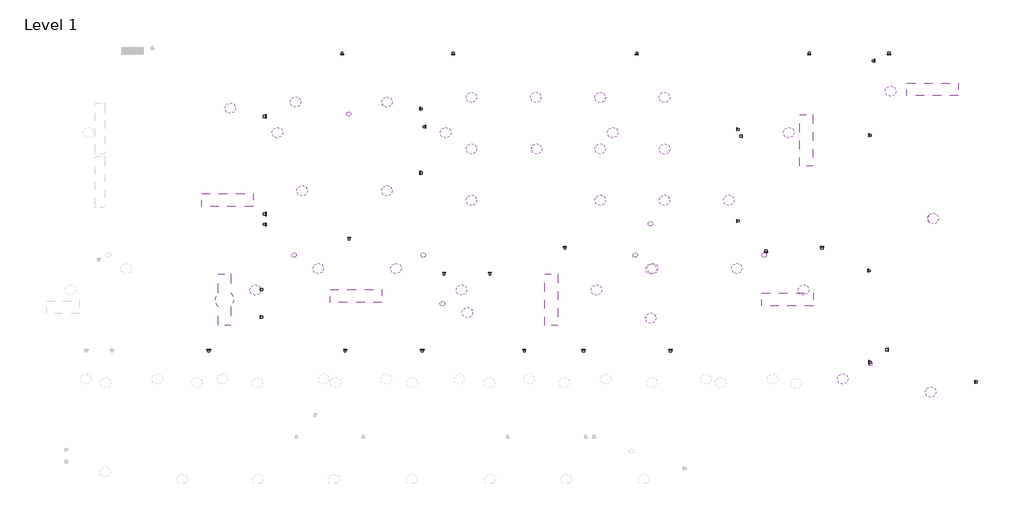
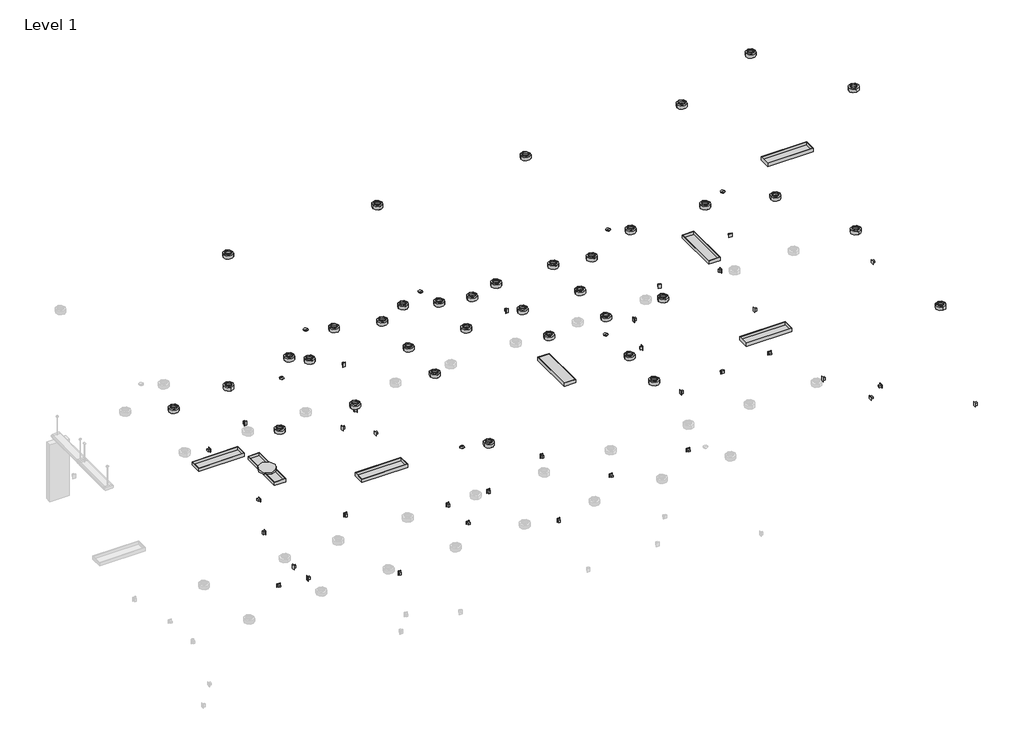
# One storey, part 3 of 3: 43 light fixtures, 22 proxies, 20 switching devices.
# Revit data of these elements (continued)
# Project information
#   Author = "F.W."
#   Classification.Facility.Description = "Mixed-Gender Dormitory"
#   Classification.Facility.Number = "11-16 27 14"
#   COBie.CreatedBy = "info@mma.ie"
#   COBie.CreatedOn = "2017-07-25T10:15:16"
#   COBie.Facility.Name = "EDTP-001"
#   COBie.Facility.Category = "11-16 27 14 : Mixed-Gender Dormitory"
#   COBie.Facility.ProjectName = "East Dormitory Project"
#   COBie.Facility.SiteName = "East Healey Street, Champaign, Illiniois USA"
#   COBie.Facility.LinearUnits = "Millimeters"
#   COBie.Facility.AreaUnits = "Square Meters"
#   COBie.Facility.VolumeUnits = "Cubic Meters"
#   COBie.Facility.CurrencyUnit = "Dollar"
#   COBie.Facility.AreaMeasurement = "Revit Default Area Calculation Method"
#   COBie.Facility.Description = "Two Story, Luxury Dormitory"
#   COBie.Facility.ProjectDescription = "One of Four Dormitories on the E.Healey Site"
#   COBie.Facility.SiteDescription = "Four Dormitories Project Site"
#   COBie.Facility.Phase = "60% Design Submission"
#   Project Issue Date = "Issue Date"
#   Project Status = "Final Issue"
#   Client Name = "Prairie Sky Consulting"
#   Project Address = "East Healey Street,\nChampaign,\nIllinois,\nUSA."
#   Project Name = "Four Dormitory Complex"
#   Project Number = "East Dormitory"
# Grids (mm)
#   "1": line (0.005, 17313.813) -> (0.005, -2035.285)
#   "A": line (-2283.993, 15250.039) -> (37015.009, 15250.039)
#   "B": line (37015.009, 12550.039) -> (-2283.993, 12550.039)
#   "C": line (37015.009, 6550.039) -> (-2283.993, 6550.039)
#   "D": line (37015.009, 2000.039) -> (-2523.993, 2000.039)
#   "E": line (37015.009, 0.039) -> (-2283.993, 0.039)
#   "2": line (1900.005, 17313.813) -> (1900.005, -2035.285)
#   "3": line (5650.005, 17313.813) -> (5650.005, -2035.285)
#   "4": line (8350.005, 17313.813) -> (8350.005, -2035.285)
#   "6": line (28050.005, -2035.285) -> (28050.005, 17313.813)
#   "8": line (34850.005, -2035.285) -> (34850.005, 17313.813)
#   "5": line (16200.005, -2035.285) -> (16200.005, 17313.813)
#   "7": line (32350.005, -2035.285) -> (32350.005, 17313.813)
# Type "M_Duplex Receptacle OFCI : GFCI"
#   Type Mark = "M_Duplex Receptacle OFCI"
#   Classification.OmniClass.23.Number = "23-35 27 11"
#   Classification.OmniClass.23.Description = "Electrical Receptacles"
#   COBie.Type.CreatedBy = "info@mma.ie"
#   COBie.Type.CreatedOn = "2017-07-25T10:15:16"
#   COBie.Type.Name = "M_Duplex Receptacle OFCI"
#   COBie.Type.Category = "23-35 27 11 : Electrical Receptacles"
#   COBie.Type.Description = "M_Duplex Receptacle OFCI_GFCI"
#   COBie.Type.AssetType = "Fixed"
#   COBie.Type.Manufacturer = ""
#   COBie.Type.ModelNumber = ""
#   Label = "GFCI"
#   Keynote = "26 27 26.C"
#   Description = "GFCI"
#   COBie.Type.ReplacementCost = 0
#   Switch Voltage = 220 V
#   Recep.Width = 69.85 mm
#   Recep.Load = 180 VA
#   Recep.Height = 114.3 mm
#   Load = 180 VA
#   Default Elevation = 1200 mm
#   COBie.Type = yes
#   Recep.Material = Stainless Steel
#   Load Classification = Receptacle
#   LEGEND = element 1211470
#   Assembly Code = ""
# Type "M_Receptacle - 220V : Standard"
#   Type Mark = "M_Receptacle - 220V"
#   Classification.OmniClass.21.Number = "21-04 50 30 50"
#   Classification.MasterFormat.Description = "Wiring Devices"
#   Classification.OmniClass.22.Number = "22-26 27 26"
#   Classification.OmniClass.21.Description = "Wiring Devices"
#   Classification.UniFormat.II.Description = "Wiring Devices"
#   Classification.MasterFormat.Number = "26 27 26"
#   Classification.OmniClass.23.Number = "23-35 27 11"
#   Classification.OmniClass.22.Description = "Wiring Devices"
#   Classification.OmniClass.23.Description = "Electrical Receptacles"
#   Classification.UniFormat.II.Number = "D5030.50"
#   COBie.Type.CreatedBy = "info@mma.ie"
#   COBie.Type.CreatedOn = "2017-07-25T10:15:16"
#   COBie.Type.Name = "M_Receptacle - 220V"
#   COBie.Type.Category = "23-35 27 11 : Electrical Receptacles"
#   COBie.Type.Description = "M_Receptacle - 220V_Standard"
#   COBie.Type.AssetType = "Fixed"
#   COBie.Type.Manufacturer = ""
#   COBie.Type.ModelNumber = ""
#   Keynote = "26 27 26.D"
#   COBie.Type.ReplacementCost = 0
#   Switch Voltage = 220 V
#   Recep.Width [instance default] = 69.85 mm
#   Recep.Load = 180 VA
#   Recep.Height [instance default] = 114.3 mm
#   Load = 180 VA
#   Default Elevation = 460 mm
#   COBie.Type = yes
#   Recep.Material = Stainless Steel
#   Load Classification = Receptacle
#   Assembly Code = ""
# Type "M_Receptacle - DATA socket : Standard"
#   Type Mark = "M_Receptacle - DATA socket"
#   Classification.OmniClass.21.Number = "21-04 50 30 50"
#   Classification.MasterFormat.Description = "Wiring Devices"
#   Classification.OmniClass.22.Number = "22-26 27 26"
#   Classification.OmniClass.21.Description = "Wiring Devices"
#   Classification.UniFormat.II.Description = "Wiring Devices"
#   Classification.MasterFormat.Number = "26 27 26"
#   Classification.OmniClass.23.Number = "23-35 27 11"
#   Classification.OmniClass.22.Description = "Wiring Devices"
#   Classification.OmniClass.23.Description = "Electrical Receptacles"
#   Classification.UniFormat.II.Number = "D5030.50"
#   COBie.Type.CreatedBy = "info@mma.ie"
#   COBie.Type.CreatedOn = "2017-07-25T10:15:16"
#   COBie.Type.Name = "M_Receptacle - DATA socket"
#   COBie.Type.Category = "23-35 27 11 : Electrical Receptacles"
#   COBie.Type.Description = "M_Receptacle - DATA socket_Standard"
#   COBie.Type.AssetType = "Fixed"
#   COBie.Type.Manufacturer = ""
#   COBie.Type.ModelNumber = ""
#   Keynote = "26 27 26.E"
#   COBie.Type.ReplacementCost = 0
#   Switch Voltage = 220 V
#   Recep.Width = 69.85 mm
#   Recep.Load = 180 VA
#   Recep.Height [instance default] = 114.3 mm
#   Load = 180 VA
#   Default Elevation = 460 mm
#   COBie.Type = yes
#   Recep.Material = Stainless Steel
#   Load Classification = Receptacle
#   Assembly Code = ""
# Type "Ceiling Light - Linear Box emergency light 300x1200mm 1Lamp 230 v : 300x1200mm(1 Lamp) - 230V"
#   Type Mark = "Ceiling Light - Linear Box emergency light 300x1200mm 1Lamp 230 v"
#   Classification.OmniClass.21.Number = "21-04 50 40 50"
#   Classification.OmniClass.21.Description = "Lighting Fixtures"
#   Classification.UniFormat.II.Description = "Lighting Fixtures"
#   Classification.OmniClass.23.Number = "23-35 47 13"
#   Classification.OmniClass.23.Description = "Emergency Lighting"
#   Classification.UniFormat.II.Number = "D5040.50"
#   COBie.Type.CreatedBy = "info@mma.ie"
#   COBie.Type.CreatedOn = "2017-07-25T10:15:16"
#   COBie.Type.Name = "Ceiling Light - Linear Box emergency light 300x1200mm 1Lamp 230 v"
#   COBie.Type.Category = "23-35 47 13 : Emergency Lighting"
#   COBie.Type.Description = "Ceiling Light - Linear Box emergency light 300x1200mm 1Lamp 230 v_300x1200mm(1 Lamp) - 230V"
#   COBie.Type.AssetType = "Fixed"
#   COBie.Type.Manufacturer = ""
#   COBie.Type.ModelNumber = ""
#   Photometric Web File = "1x41T12.ies"
#   Lamp = "T-12"
#   Keynote = "26 52 00.A"
#   Assembly Code = "D5020210"
#   COBie.Type.ReplacementCost = 0
#   Width 1 = 150 mm
#   Wattage = 40 W
#   built-in parameter 1150110 = 1 (stored number, unit not read)
#   built-in parameter 1114217 = 0.88 (stored number, unit not read)
#   built-in parameter 1150109 = 1 (stored number, unit not read)
#   built-in parameter 1150113 = 1 (stored number, unit not read)
#   Tilt Angle = -90.00°
#   Lumens = 3150 lm
#   built-in parameter 1150115 = 1 (stored number, unit not read)
#   built-in parameter 1150105 = 250.669 (stored number, unit not read)
#   Length1 = 600 mm
#   built-in parameter 1150112 = 1 (stored number, unit not read)
#   built-in parameter 1150114 = 1 (stored number, unit not read)
#   built-in parameter 1150107 = 4230 (stored number, unit not read)
#   built-in parameter 1150106 = 2.50669 (stored number, unit not read)
#   Emit from Rectangle Width = 274 mm
#   Emit from Rectangle Length = 1174 mm
#   built-in parameter 1150104 = 7.31611 (stored number, unit not read)
#   Default Elevation = 1200 mm
#   C.L.E - Width = 300 mm
#   C.L.E - Length = 1200 mm
#   C.L.E - Depth = 88.9 mm
#   Box Width = 300 mm
#   Box Length = 1200 mm
#   Ballast Voltage = 230 V
#   built-in parameter 1114218 = 0.88 (stored number, unit not read)
#   built-in parameter 1150133 = 10 (stored number, unit not read)
#   Apparent Load = 40 VA
#   COBie.Type = yes
#   built-in parameter 1150134 = 8
#   built-in parameter 1150137 = 1
#   Color Filter = 16777215
#   built-in parameter 1140040 [instance default] = 1
#   Ballast Number of Poles = 1
#   black = Phase - Demo
#   Load Classification = Lighting - Dwelling Unit
#   Light Box Material = Metal - Paint Finish - Ivory, Glossy
#   Diffuser Material = Glass - White, High Luminance
#   Emit Shape Visible in Rendering = no
#   Dimming Lamp Color Temperature Shift = (empty or 0)
# Type "Ceiling Light - Linear Box 300x1200 : 0300x1200mm(1 Lamp) - 230V"
#   Type Mark = "Ceiling Light - Linear Box 300x1200"
#   Classification.OmniClass.23.Number = "23-35 47 11"
#   Classification.OmniClass.23.Description = "Lighting Fixtures"
#   COBie.Type.CreatedBy = "info@mma.ie"
#   COBie.Type.CreatedOn = "2017-07-25T10:15:16"
#   COBie.Type.Name = "Ceiling Light - Linear Box 300x1200"
#   COBie.Type.Category = "23-35 47 11 : Lighting Fixtures"
#   COBie.Type.Description = "Ceiling Light - Linear Box 300x1200_0300x1200mm(1 Lamp) - 230V"
#   COBie.Type.AssetType = "Fixed"
#   COBie.Type.Manufacturer = ""
#   COBie.Type.ModelNumber = ""
#   Photometric Web File = "1x41T12.ies"
#   Lamp = "T-12"
#   Keynote = "26 51 13.A"
#   Assembly Code = "D5020210"
#   COBie.Type.ReplacementCost = 0
#   Width 1 = 150 mm
#   Wattage = 40 W
#   built-in parameter 1150110 = 1 (stored number, unit not read)
#   built-in parameter 1114217 = 0.88 (stored number, unit not read)
#   built-in parameter 1150109 = 1 (stored number, unit not read)
#   built-in parameter 1150113 = 1 (stored number, unit not read)
#   Tilt Angle = -90.00°
#   Lumens = 3150 lm
#   built-in parameter 1150115 = 1 (stored number, unit not read)
#   built-in parameter 1150105 = 250.669 (stored number, unit not read)
#   Length1 = 600 mm
#   built-in parameter 1150112 = 1 (stored number, unit not read)
#   built-in parameter 1150114 = 1 (stored number, unit not read)
#   built-in parameter 1150107 = 4230 (stored number, unit not read)
#   built-in parameter 1150106 = 2.50669 (stored number, unit not read)
#   Emit from Rectangle Width = 274 mm
#   Emit from Rectangle Length = 1174 mm
#   built-in parameter 1150104 = 7.31611 (stored number, unit not read)
#   Default Elevation = 1200 mm
#   C.L. Width = 300 mm
#   C.L. Length = 1200 mm
#   C.L. Depth = 88.9 mm
#   Ballast Voltage = 230 V
#   built-in parameter 1114218 = 0.88 (stored number, unit not read)
#   built-in parameter 1150133 = 10 (stored number, unit not read)
#   Apparent Load = 40 VA
#   COBie.Type = yes
#   built-in parameter 1150134 = 8
#   built-in parameter 1150137 = 1
#   Color Filter = 16777215
#   built-in parameter 1140040 [instance default] = 1
#   Ballast Number of Poles = 1
#   Load Classification = Lighting - Dwelling Unit
#   Light Box Material = Metal - Paint Finish - Ivory, Glossy
#   Diffuser Material = Glass - White, High Luminance
#   BLACK = Phase - Demo
#   Emit Shape Visible in Rendering = no
#   Dimming Lamp Color Temperature Shift = (empty or 0)
# Type "CeilingLight-RoundEmergency : 100W - 230V"
#   Type Mark = "CeilingLight-RoundEmergencyB"
#   Classification.OmniClass.21.Number = "21-04 50 40 50"
#   Classification.OmniClass.21.Description = "Lighting Fixtures"
#   Classification.UniFormat.II.Description = "Lighting Fixtures"
#   Classification.OmniClass.23.Number = "23-35 47 13"
#   Classification.OmniClass.23.Description = "Emergency Lighting"
#   Classification.UniFormat.II.Number = "D5040.50"
#   COBie.Type.CreatedBy = "info@mma.ie"
#   COBie.Type.CreatedOn = "2017-07-25T10:15:16"
#   COBie.Type.Name = "CeilingLight-RoundEmergencyB"
#   COBie.Type.Category = "23-35 47 13 : Emergency Lighting"
#   COBie.Type.Description = "CeilingLight-RoundEmergency_100W - 230V"
#   COBie.Type.AssetType = "Fixed"
#   COBie.Type.Manufacturer = ""
#   COBie.Type.ModelNumber = ""
#   Keynote = "26 52 00.B"
#   Lamp = "A-19"
#   Photometric Web File = "CLFR1A21.ies"
#   Assembly Code = "D5020220"
#   COBie.Type.ReplacementCost = 0
#   Wattage = 100 W
#   built-in parameter 1150110 = 1 (stored number, unit not read)
#   built-in parameter 1150109 = 1 (stored number, unit not read)
#   built-in parameter 1150113 = 1 (stored number, unit not read)
#   Tilt Angle = -90.00°
#   built-in parameter 1150115 = 1 (stored number, unit not read)
#   built-in parameter 1150105 = 139.261 (stored number, unit not read)
#   built-in parameter 1150112 = 1 (stored number, unit not read)
#   built-in parameter 1150114 = 1 (stored number, unit not read)
#   built-in parameter 1150107 = 2800 (stored number, unit not read)
#   built-in parameter 1150106 = 1.39261 (stored number, unit not read)
#   Emit from Circle Diameter = 254 mm
#   built-in parameter 1150104 = 1.6258 (stored number, unit not read)
#   E.C.L. Efficacy = 17.5 lm/W
#   E.C.L. Diameter = 254 mm
#   Lumens = 1750 lm
#   built-in parameter 1114217 = 1 (stored number, unit not read)
#   Default Elevation = 1200 mm
#   Ballast Voltage = 230 V
#   built-in parameter 1114218 = 1 (stored number, unit not read)
#   built-in parameter 1150133 = 10 (stored number, unit not read)
#   Apparent Load = 100 VA
#   COBie.Type = yes
#   built-in parameter 1150134 = 4
#   built-in parameter 1150137 = 1
#   Color Filter = 16777215
#   built-in parameter 1140040 [instance default] = 1
#   Ballast Number of Poles = 1
#   black = Glass - White, High Luminance
#   Load Classification = Lighting - Dwelling Unit
#   Light Box Material = Metal - Paint Finish - Dark Grey, Matt
#   E.C.L. Material = Metal - Paint Finish - Dark Grey, Matt
#   Diffuser Material = Glass - White, High Luminance
#   Emit Shape Visible in Rendering = no
#   Dimming Lamp Color Temperature Shift = (empty or 0)
# Type "CeilingLight-RoundEmergency : 60W - 230V"
#   Type Mark = "CeilingLight-RoundEmergencyA"
#   Classification.OmniClass.21.Number = "21-04 50 40 50"
#   Classification.OmniClass.21.Description = "Lighting Fixtures"
#   Classification.UniFormat.II.Description = "Lighting Fixtures"
#   Classification.OmniClass.23.Number = "23-35 47 13"
#   Classification.OmniClass.23.Description = "Emergency Lighting"
#   Classification.UniFormat.II.Number = "D5040.50"
#   COBie.Type.CreatedBy = "info@mma.ie"
#   COBie.Type.CreatedOn = "2017-07-25T10:15:16"
#   COBie.Type.Name = "CeilingLight-RoundEmergencyA"
#   COBie.Type.Category = "23-35 47 13 : Emergency Lighting"
#   COBie.Type.Description = "CeilingLight-RoundEmergency_60W - 230V"
#   COBie.Type.AssetType = "Fixed"
#   COBie.Type.Manufacturer = ""
#   COBie.Type.ModelNumber = ""
#   Keynote = "26 52 00.B"
#   Lamp = "A-19"
#   Photometric Web File = "CLFR1A19.ies"
#   Assembly Code = "D5020220"
#   COBie.Type.ReplacementCost = 0
#   Wattage = 60 W
#   built-in parameter 1150110 = 1 (stored number, unit not read)
#   built-in parameter 1150109 = 1 (stored number, unit not read)
#   built-in parameter 1150113 = 1 (stored number, unit not read)
#   Tilt Angle = -90.00°
#   built-in parameter 1150115 = 1 (stored number, unit not read)
#   built-in parameter 1150105 = 68.0387 (stored number, unit not read)
#   built-in parameter 1150112 = 1 (stored number, unit not read)
#   built-in parameter 1150114 = 1 (stored number, unit not read)
#   built-in parameter 1150107 = 2800 (stored number, unit not read)
#   built-in parameter 1150106 = 0.680387 (stored number, unit not read)
#   Emit from Circle Diameter = 254 mm
#   built-in parameter 1150104 = 1.32387 (stored number, unit not read)
#   E.C.L. Efficacy = 17.5 lm/W
#   E.C.L. Diameter = 254 mm
#   Lumens = 855 lm
#   built-in parameter 1114217 = 1 (stored number, unit not read)
#   Default Elevation = 1200 mm
#   Ballast Voltage = 230 V
#   built-in parameter 1114218 = 1 (stored number, unit not read)
#   built-in parameter 1150133 = 10 (stored number, unit not read)
#   Apparent Load = 60 VA
#   COBie.Type = yes
#   built-in parameter 1150134 = 4
#   built-in parameter 1150137 = 1
#   Color Filter = 16777215
#   built-in parameter 1140040 [instance default] = 1
#   Ballast Number of Poles = 1
#   black = Phase-Demo
#   Load Classification = Lighting - Dwelling Unit
#   Light Box Material = Metal - Paint Finish - Dark Grey, Matt
#   E.C.L. Material = Metal - Paint Finish - Dark Grey, Matt
#   Diffuser Material = Glass - White, High Luminance
#   Emit Shape Visible in Rendering = no
#   Dimming Lamp Color Temperature Shift = (empty or 0)
# Type "CeilingOccupancySensor : 450"
#   Type Mark = "CeilingOccupancySensor"
#   Classification.OmniClass.21.Number = "21-04 50 40 10"
#   Classification.OmniClass.21.Description = "Lighting Control"
#   Classification.UniFormat.II.Description = "Lighting Control"
#   Classification.OmniClass.23.Number = "23-29 11 23 17"
#   Classification.OmniClass.23.Description = "Intrusion Detection Photoelectric Sensors"
#   Classification.UniFormat.II.Number = "D5040.10"
#   COBie.Type.CreatedBy = "info@mma.ie"
#   COBie.Type.CreatedOn = "2017-07-25T10:15:16"
#   COBie.Type.Name = "CeilingOccupancySensor"
#   COBie.Type.Category = "23-29 11 23 17 : Intrusion Detection Photoelectric Sensors"
#   COBie.Type.Description = "CeilingOccupancySensor_450"
#   COBie.Type.AssetType = "Fixed"
#   COBie.Type.Manufacturer = ""
#   COBie.Type.ModelNumber = ""
#   Voltage Comments = "20-24VDC"
#   Series = ""
#   Product URL = ""
#   Keynote = "28 16 19.A"
#   Copyright = ""
#   CADworks URL = ""
#   C.O.S. Material = "Plastic-White-Gloss"
#   Assembly Code = "D5030800"
#   COBie.Type.ReplacementCost = 0
#   Switch Voltage = 230 V
#   Nominal Width = 114.3 mm
#   Nominal Length = 114.3 mm
#   Nominal Depth = 35.52 mm
#   Minor Motion Detection = 1981.2 mm
#   Major Motion Detection = 3657.6 mm
#   Field of View = 360.00°
#   Coverage = 41.8064 m²
#   C.O.S. Field of View = 360.00°
#   C.O.S. Coverage = 41.8064 m²
#   COBie.Type = yes
#   Light Source [instance default] = yes
#   Infrared Minor Motion [instance default] = no
#   Infrared Major Motion [instance default] = no
#   Ballast Number of Poles = 1
#   Sensor Material = Plastic-White-Gloss
#   URL = ""
#   Type Comments = ""
#   Model = ""
#   Manufacturer = ""
#   Description = (empty or 0)
#   Default Elevation = 0
# Type "Lighting Switches One Way : One Way Switch"
#   Type Mark = "Lighting Switches One Way"
#   Classification.OmniClass.21.Number = "21-04 50 40 10"
#   Classification.OmniClass.21.Description = "Lighting Control"
#   Classification.UniFormat.II.Description = "Lighting Control"
#   Classification.OmniClass.23.Number = "23-35 37 00"
#   Classification.OmniClass.23.Description = "Electrical Switches"
#   Classification.UniFormat.II.Number = "D5040.10"
#   COBie.Type.CreatedBy = "info@mma.ie"
#   COBie.Type.CreatedOn = "2017-07-25T10:15:16"
#   COBie.Type.Name = "Lighting Switches One Way"
#   COBie.Type.Category = "23-35 37 00 : Electrical Switches"
#   COBie.Type.Description = "Lighting Switches One Way_One Way Switch"
#   COBie.Type.AssetType = "Fixed"
#   COBie.Type.Manufacturer = ""
#   COBie.Type.ModelNumber = ""
#   Label = ""
#   Keynote = "26 36 13.A"
#   COBie.Type.ReplacementCost = 0
#   Switch Voltage [instance default] = 230 V
#   Default Elevation = 1200 mm
#   Apparent Load = 0 VA
#   1.W.S. Width = 86 mm
#   1.W.S. Height = 86 mm
#   1.W.S. Depth = 59 mm
#   COBie.Type = yes
#   Visibility 7 = no
#   Visibility 6 = no
#   Visibility 5 = yes
#   Visibility 4 = no
#   Visibility 3 = no
#   Visibility 2 = no
#   Visibility 1 = no
#   Ballast Number of Poles = 1
#   Load Classification = Other
#   1.W.S. Material = Metal - Chrome
# Type "Lighting Switches Two Way : Two Way Switch"
#   Type Mark = "Lighting Switches Two Way"
#   Classification.OmniClass.23.Number = "23-35 37 00"
#   Classification.OmniClass.23.Description = "Electrical Switches"
#   COBie.Type.CreatedBy = "info@mma.ie"
#   COBie.Type.CreatedOn = "2017-07-25T10:15:16"
#   COBie.Type.Name = "Lighting Switches Two Way"
#   COBie.Type.Category = "23-35 37 00 : Electrical Switches"
#   COBie.Type.Description = "Lighting Switches Two Way_Two Way Switch"
#   COBie.Type.AssetType = "Fixed"
#   COBie.Type.Manufacturer = ""
#   COBie.Type.ModelNumber = ""
#   Label = ""
#   Keynote = "26 36 13.B"
#   COBie.Type.ReplacementCost = 0
#   Switch Voltage [instance default] = 230 V
#   Default Elevation = 1200 mm
#   Apparent Load = 0 VA
#   2.W.S. Width = 86 mm
#   2.W.S. Height = 86 mm
#   2.W.S. Depth = 59 mm
#   COBie.Type = yes
#   Visibility 7 = no
#   Visibility 6 = no
#   Visibility 5 = yes
#   Visibility 4 = no
#   Visibility 3 = no
#   Visibility 2 = no
#   Visibility 1 = no
#   Ballast Number of Poles = 1
#   Load Classification = Other
#   2.W.S. Material = Metal - Chrome
# Element 1 (IfcBuildingElementProxy, "M_Duplex Receptacle OFCI : GFCI")
#   Mark = "4"
#   COBie.CreatedBy = "info@mma.ie"
#   COBie.CreatedOn = "2017-07-25T10:15:16"
#   COBie.Component.Name = "M_Duplex Receptacle OFCI_4"
#   COBie.Component.Space = "112"
#   COBie.Component.Description = "M_Duplex Receptacle OFCI: GFCI"
#   Notes = "n/a"
#   COBie = yes
#   Phase Created = New Construction
# Element 2 (IfcBuildingElementProxy, "M_Duplex Receptacle OFCI : GFCI")
#   Mark = "5"
#   COBie.CreatedBy = "info@mma.ie"
#   COBie.CreatedOn = "2017-07-25T10:15:16"
#   COBie.Component.Name = "M_Duplex Receptacle OFCI_5"
#   COBie.Component.Space = "112"
#   COBie.Component.Description = "M_Duplex Receptacle OFCI: GFCI"
#   Notes = "n/a"
#   COBie = yes
#   Phase Created = New Construction
# Element 3 (IfcBuildingElementProxy, "M_Duplex Receptacle OFCI : GFCI")
#   Mark = "6"
#   COBie.CreatedBy = "info@mma.ie"
#   COBie.CreatedOn = "2017-07-25T10:15:16"
#   COBie.Component.Name = "M_Duplex Receptacle OFCI_6"
#   COBie.Component.Space = "112"
#   COBie.Component.Description = "M_Duplex Receptacle OFCI: GFCI"
#   Notes = "n/a"
#   COBie = yes
#   Phase Created = New Construction
# Element 4 (IfcBuildingElementProxy, "M_Duplex Receptacle OFCI : GFCI")
#   Mark = "7"
#   COBie.CreatedBy = "info@mma.ie"
#   COBie.CreatedOn = "2017-07-25T10:15:16"
#   COBie.Component.Name = "M_Duplex Receptacle OFCI_7"
#   COBie.Component.Space = "112"
#   COBie.Component.Description = "M_Duplex Receptacle OFCI: GFCI"
#   Notes = "n/a"
#   COBie = yes
#   Phase Created = New Construction
# Element 5 (IfcBuildingElementProxy, "M_Receptacle - 220V : Standard")
#   Mark = "43"
#   COBie.CreatedBy = "info@mma.ie"
#   COBie.CreatedOn = "2017-07-25T10:15:16"
#   COBie.Component.Name = "M_Receptacle - 220V_43"
#   COBie.Component.Space = "110"
#   COBie.Component.Description = "M_Receptacle - 220V: Standard"
#   Notes = "n/a"
#   COBie = yes
#   Phase Created = New Construction
# Element 6 (IfcBuildingElementProxy, "M_Receptacle - 220V : Standard")
#   Mark = "60"
#   COBie.CreatedBy = "info@mma.ie"
#   COBie.CreatedOn = "2017-07-25T10:15:16"
#   COBie.Component.Name = "M_Receptacle - 220V_60"
#   COBie.Component.Space = "108"
#   COBie.Component.Description = "M_Receptacle - 220V: Standard"
#   Notes = "n/a"
#   COBie = yes
#   Phase Created = New Construction
# Element 7 (IfcBuildingElementProxy, "M_Receptacle - 220V : Standard")
#   Mark = "61"
#   COBie.CreatedBy = "info@mma.ie"
#   COBie.CreatedOn = "2017-07-25T10:15:16"
#   COBie.Component.Name = "M_Receptacle - 220V_61"
#   COBie.Component.Space = "108"
#   COBie.Component.Description = "M_Receptacle - 220V: Standard"
#   Notes = "n/a"
#   COBie = yes
#   Phase Created = New Construction
# Element 8 (IfcBuildingElementProxy, "M_Receptacle - 220V : Standard")
#   Mark = "62"
#   COBie.CreatedBy = "info@mma.ie"
#   COBie.CreatedOn = "2017-07-25T10:15:16"
#   COBie.Component.Name = "M_Receptacle - 220V_62"
#   COBie.Component.Space = "108"
#   COBie.Component.Description = "M_Receptacle - 220V: Standard"
#   Notes = "n/a"
#   COBie = yes
#   Phase Created = New Construction
# Element 9 (IfcBuildingElementProxy, "M_Receptacle - 220V : Standard")
#   Mark = "63"
#   COBie.CreatedBy = "info@mma.ie"
#   COBie.CreatedOn = "2017-07-25T10:15:16"
#   COBie.Component.Name = "M_Receptacle - 220V_63"
#   COBie.Component.Space = "108"
#   COBie.Component.Description = "M_Receptacle - 220V: Standard"
#   Notes = "n/a"
#   COBie = yes
#   Phase Created = New Construction
# Element 10 (IfcBuildingElementProxy, "M_Receptacle - 220V : Standard")
#   Mark = "64"
#   COBie.CreatedBy = "info@mma.ie"
#   COBie.CreatedOn = "2017-07-25T10:15:16"
#   COBie.Component.Name = "M_Receptacle - 220V_64"
#   COBie.Component.Space = "112"
#   COBie.Component.Description = "M_Receptacle - 220V: Standard"
#   Notes = "n/a"
#   COBie = yes
#   Phase Created = New Construction
# Element 11 (IfcBuildingElementProxy, "M_Receptacle - 220V : Standard")
#   Mark = "65"
#   COBie.CreatedBy = "info@mma.ie"
#   COBie.CreatedOn = "2017-07-25T10:15:16"
#   COBie.Component.Name = "M_Receptacle - 220V_65"
#   COBie.Component.Space = "112"
#   COBie.Component.Description = "M_Receptacle - 220V: Standard"
#   Notes = "n/a"
#   COBie = yes
#   Phase Created = New Construction
# Element 12 (IfcBuildingElementProxy, "M_Receptacle - 220V : Standard")
#   Mark = "67"
#   COBie.CreatedBy = "info@mma.ie"
#   COBie.CreatedOn = "2017-07-25T10:15:16"
#   COBie.Component.Name = "M_Receptacle - 220V_67"
#   COBie.Component.Space = "113"
#   COBie.Component.Description = "M_Receptacle - 220V: Standard"
#   Notes = "n/a"
#   COBie = yes
#   Phase Created = New Construction
# Element 13 (IfcBuildingElementProxy, "M_Receptacle - 220V : Standard")
#   Mark = "68"
#   COBie.CreatedBy = "info@mma.ie"
#   COBie.CreatedOn = "2017-07-25T10:15:16"
#   COBie.Component.Name = "M_Receptacle - 220V_68"
#   COBie.Component.Space = "113"
#   COBie.Component.Description = "M_Receptacle - 220V: Standard"
#   Notes = "n/a"
#   COBie = yes
#   Phase Created = New Construction
# Element 14 (IfcBuildingElementProxy, "M_Receptacle - 220V : Standard")
#   Mark = "69"
#   COBie.CreatedBy = "info@mma.ie"
#   COBie.CreatedOn = "2017-07-25T10:15:16"
#   COBie.Component.Name = "M_Receptacle - 220V_69"
#   COBie.Component.Space = "113"
#   COBie.Component.Description = "M_Receptacle - 220V: Standard"
#   Notes = "n/a"
#   COBie = yes
#   Phase Created = New Construction
# Element 15 (IfcBuildingElementProxy, "M_Receptacle - 220V : Standard")
#   Mark = "70"
#   COBie.CreatedBy = "info@mma.ie"
#   COBie.CreatedOn = "2017-07-25T10:15:16"
#   COBie.Component.Name = "M_Receptacle - 220V_70"
#   COBie.Component.Space = "115"
#   COBie.Component.Description = "M_Receptacle - 220V: Standard"
#   Notes = "n/a"
#   COBie = yes
#   Phase Created = New Construction
# Element 16 (IfcBuildingElementProxy, "M_Receptacle - 220V : Standard")
#   Mark = "71"
#   COBie.CreatedBy = "info@mma.ie"
#   COBie.CreatedOn = "2017-07-25T10:15:16"
#   COBie.Component.Name = "M_Receptacle - 220V_71"
#   COBie.Component.Space = "116"
#   COBie.Component.Description = "M_Receptacle - 220V: Standard"
#   Notes = "n/a"
#   COBie = yes
#   Phase Created = New Construction
# Element 17 (IfcBuildingElementProxy, "M_Receptacle - 220V : Standard")
#   Mark = "82"
#   COBie.CreatedBy = "info@mma.ie"
#   COBie.CreatedOn = "2017-07-25T10:15:16"
#   COBie.Component.Name = "M_Receptacle - 220V_82"
#   COBie.Component.Space = "111"
#   COBie.Component.Description = "M_Receptacle - 220V: Standard"
#   Notes = "n/a"
#   COBie = yes
#   Phase Created = New Construction
# Element 18 (IfcBuildingElementProxy, "M_Receptacle - 220V : Standard")
#   Mark = "83"
#   COBie.CreatedBy = "info@mma.ie"
#   COBie.CreatedOn = "2017-07-25T10:15:16"
#   COBie.Component.Name = "M_Receptacle - 220V_83"
#   COBie.Component.Space = "114"
#   COBie.Component.Description = "M_Receptacle - 220V: Standard"
#   Notes = "n/a"
#   COBie = yes
#   Phase Created = New Construction
# Element 19 (IfcBuildingElementProxy, "M_Receptacle - 220V : Standard")
#   Mark = "84"
#   COBie.CreatedBy = "info@mma.ie"
#   COBie.CreatedOn = "2017-07-25T10:15:16"
#   COBie.Component.Name = "M_Receptacle - 220V_84"
#   COBie.Component.Space = "109"
#   COBie.Component.Description = "M_Receptacle - 220V: Standard"
#   Notes = "n/a"
#   COBie = yes
#   Phase Created = New Construction
# Element 20 (IfcBuildingElementProxy, "M_Receptacle - 220V : Standard")
#   Mark = "85"
#   COBie.CreatedBy = "info@mma.ie"
#   COBie.CreatedOn = "2017-07-25T10:15:16"
#   COBie.Component.Name = "M_Receptacle - 220V_85"
#   COBie.Component.Space = "112"
#   COBie.Component.Description = "M_Receptacle - 220V: Standard"
#   Notes = "n/a"
#   COBie = yes
#   Phase Created = New Construction
# Element 21 (IfcBuildingElementProxy, "M_Receptacle - 220V : Standard")
#   Mark = "66"
#   COBie.CreatedBy = "info@mma.ie"
#   COBie.CreatedOn = "2017-07-25T10:15:16"
#   COBie.Component.Name = "M_Receptacle - 220V_66"
#   COBie.Component.Space = "112"
#   COBie.Component.Description = "M_Receptacle - 220V: Standard"
#   Notes = "n/a"
#   COBie = yes
#   Phase Created = New Construction
# Element 22 (IfcBuildingElementProxy, "M_Receptacle - DATA socket : Standard")
#   Mark = "17"
#   COBie.CreatedBy = "info@mma.ie"
#   COBie.CreatedOn = "2017-07-25T10:15:16"
#   COBie.Component.Name = "M_Receptacle - DATA socket_17"
#   COBie.Component.Space = "109"
#   COBie.Component.Description = "M_Receptacle - DATA socket: Standard"
#   Notes = "n/a"
#   COBie = yes
#   Phase Created = New Construction
# Element 23 (IfcLightFixture, "Ceiling Light - Linear Box emergency light 300x1200mm 1Lamp 230 v : 300x1200mm(1 Lamp) - 230V")
#   Comments = "Light"
#   Mark = "3"
#   COBie.CreatedBy = "info@mma.ie"
#   COBie.CreatedOn = "2017-07-25T10:15:16"
#   COBie.Component.Name = "Ceiling Light - Linear Box emergency light 300x1200mm 1Lamp 230 v_3"
#   COBie.Component.Space = "109"
#   COBie.Component.Description = "Ceiling Light - Linear Box emergency light 300x1200mm 1Lamp 230 v: 0300x1200mm(1 Lamp) - 230V"
#   Notes = "n/a"
#   Floor Level = "Level 1"
#   COBie = yes
#   built-in parameter 1140040 = 1
#   Phase Created = New Construction
#   Materials on its faces: "Phase - Demo", "Glass - White, High Luminance"
# Element 24 (IfcLightFixture, "Ceiling Light - Linear Box 300x1200 : 0300x1200mm(1 Lamp) - 230V")
#   Comments = "Light"
#   Mark = "1"
#   COBie.CreatedBy = "info@mma.ie"
#   COBie.CreatedOn = "2017-07-25T10:15:16"
#   COBie.Component.Name = "Ceiling Light - Linear Box 300x1200_1"
#   COBie.Component.Space = "110"
#   COBie.Component.Description = "Ceiling Light - Linear Box 300x1200: 0300x1200mm(1 Lamp) - 230V"
#   Notes = "n/a"
#   Floor Level = "Level 1"
#   COBie = yes
#   built-in parameter 1140040 = 1
#   Phase Created = New Construction
#   Materials on its faces: "Phase - Demo", "Glass - White, High Luminance"
# Element 25 (IfcLightFixture, "Ceiling Light - Linear Box 300x1200 : 0300x1200mm(1 Lamp) - 230V")
#   Comments = "Light"
#   Mark = "2"
#   COBie.CreatedBy = "info@mma.ie"
#   COBie.CreatedOn = "2017-07-25T10:15:16"
#   COBie.Component.Name = "Ceiling Light - Linear Box 300x1200_2"
#   COBie.Component.Space = "113"
#   COBie.Component.Description = "Ceiling Light - Linear Box 300x1200: 0300x1200mm(1 Lamp) - 230V"
#   Notes = "n/a"
#   Floor Level = "Level 1"
#   COBie = yes
#   built-in parameter 1140040 = 1
#   Phase Created = New Construction
#   Materials on its faces: "Phase - Demo", "Glass - White, High Luminance"
# Element 26 (IfcLightFixture, "Ceiling Light - Linear Box 300x1200 : 0300x1200mm(1 Lamp) - 230V")
#   Comments = "Light"
#   Mark = "9"
#   COBie.CreatedBy = "info@mma.ie"
#   COBie.CreatedOn = "2017-07-25T10:15:16"
#   COBie.Component.Name = "Ceiling Light - Linear Box 300x1200_9"
#   COBie.Component.Space = "213"
#   COBie.Component.Description = "Ceiling Light - Linear Box 300x1200: 0300x1200mm(1 Lamp) - 230V"
#   Notes = "n/a"
#   Floor Level = "Level 1"
#   COBie = yes
#   built-in parameter 1140040 = 1
#   Phase Created = New Construction
#   Materials on its faces: "Phase - Demo", "Glass - White, High Luminance"
# Element 27 (IfcLightFixture, "Ceiling Light - Linear Box 300x1200 : 0300x1200mm(1 Lamp) - 230V")
#   Comments = "Light"
#   Mark = "10"
#   COBie.CreatedBy = "info@mma.ie"
#   COBie.CreatedOn = "2017-07-25T10:15:16"
#   COBie.Component.Name = "Ceiling Light - Linear Box 300x1200_10"
#   COBie.Component.Space = "114"
#   COBie.Component.Description = "Ceiling Light - Linear Box 300x1200: 0300x1200mm(1 Lamp) - 230V"
#   Notes = "n/a"
#   Floor Level = "Level 1"
#   COBie = yes
#   built-in parameter 1140040 = 1
#   Phase Created = New Construction
#   Materials on its faces: "Phase - Demo", "Glass - White, High Luminance"
# Element 28 (IfcLightFixture, "Ceiling Light - Linear Box 300x1200 : 0300x1200mm(1 Lamp) - 230V")
#   Comments = "Light"
#   Mark = "11"
#   COBie.CreatedBy = "info@mma.ie"
#   COBie.CreatedOn = "2017-07-25T10:15:16"
#   COBie.Component.Name = "Ceiling Light - Linear Box 300x1200_11"
#   COBie.Component.Space = "107"
#   COBie.Component.Description = "Ceiling Light - Linear Box 300x1200: 0300x1200mm(1 Lamp) - 230V"
#   Notes = "n/a"
#   Floor Level = "Level 1"
#   COBie = yes
#   built-in parameter 1140040 = 1
#   Phase Created = New Construction
#   Materials on its faces: "Phase - Demo", "Glass - White, High Luminance"
# Element 29 (IfcLightFixture, "Ceiling Light - Linear Box 300x1200 : 0300x1200mm(1 Lamp) - 230V")
#   Comments = "Light"
#   Mark = "13"
#   COBie.CreatedBy = "info@mma.ie"
#   COBie.CreatedOn = "2017-07-25T10:15:16"
#   COBie.Component.Name = "Ceiling Light - Linear Box 300x1200_13"
#   COBie.Component.Space = "115"
#   COBie.Component.Description = "Ceiling Light - Linear Box 300x1200: 0300x1200mm(1 Lamp) - 230V"
#   Notes = "n/a"
#   Floor Level = "Level 1"
#   COBie = yes
#   built-in parameter 1140040 = 1
#   Phase Created = New Construction
#   Materials on its faces: "Phase - Demo", "Glass - White, High Luminance"
# Element 30 (IfcLightFixture, "CeilingLight-RoundEmergency : 100W - 230V")
#   Comments = "Light"
#   Mark = "4"
#   COBie.CreatedBy = "info@mma.ie"
#   COBie.CreatedOn = "2017-07-25T10:15:16"
#   COBie.Component.Name = "CeilingLight-RoundEmergencyB_4"
#   COBie.Component.Space = "106"
#   COBie.Component.Description = "CeilingLight-RoundEmergency: 100W - 230V"
#   Notes = "n/a"
#   Floor Level = "Level 1"
#   COBie = yes
#   built-in parameter 1140040 = 1
#   Phase Created = New Construction
#   Materials on its faces: "Glass - White, High Luminance", "Metal - Paint Finish - Dark Grey, Matt"
# Element 31 (IfcLightFixture, "CeilingLight-RoundEmergency : 100W - 230V")
#   Comments = "Light"
#   Mark = "5"
#   COBie.CreatedBy = "info@mma.ie"
#   COBie.CreatedOn = "2017-07-25T10:15:16"
#   COBie.Component.Name = "CeilingLight-RoundEmergencyB_5"
#   COBie.Component.Space = "108"
#   COBie.Component.Description = "CeilingLight-RoundEmergency: 100W - 230V"
#   Notes = "n/a"
#   Floor Level = "Level 1"
#   COBie = yes
#   built-in parameter 1140040 = 1
#   Phase Created = New Construction
#   Materials on its faces: "Glass - White, High Luminance", "Metal - Paint Finish - Dark Grey, Matt"
# Element 32 (IfcLightFixture, "CeilingLight-RoundEmergency : 100W - 230V")
#   Comments = "Light"
#   Mark = "6"
#   COBie.CreatedBy = "info@mma.ie"
#   COBie.CreatedOn = "2017-07-25T10:15:16"
#   COBie.Component.Name = "CeilingLight-RoundEmergencyB_6"
#   COBie.Component.Space = "108"
#   COBie.Component.Description = "CeilingLight-RoundEmergency: 100W - 230V"
#   Notes = "n/a"
#   Floor Level = "Level 1"
#   COBie = yes
#   built-in parameter 1140040 = 1
#   Phase Created = New Construction
#   Materials on its faces: "Glass - White, High Luminance", "Metal - Paint Finish - Dark Grey, Matt"
# Element 33 (IfcLightFixture, "CeilingLight-RoundEmergency : 100W - 230V")
#   Comments = "Light"
#   Mark = "7"
#   COBie.CreatedBy = "info@mma.ie"
#   COBie.CreatedOn = "2017-07-25T10:15:16"
#   COBie.Component.Name = "CeilingLight-RoundEmergencyB_7"
#   COBie.Component.Space = "108"
#   COBie.Component.Description = "CeilingLight-RoundEmergency: 100W - 230V"
#   Notes = "n/a"
#   Floor Level = "Level 1"
#   COBie = yes
#   built-in parameter 1140040 = 1
#   Phase Created = New Construction
#   Materials on its faces: "Glass - White, High Luminance", "Metal - Paint Finish - Dark Grey, Matt"
# Element 34 (IfcLightFixture, "CeilingLight-RoundEmergency : 100W - 230V")
#   Comments = "Light"
#   Mark = "8"
#   COBie.CreatedBy = "info@mma.ie"
#   COBie.CreatedOn = "2017-07-25T10:15:16"
#   COBie.Component.Name = "CeilingLight-RoundEmergencyB_8"
#   COBie.Component.Space = "108"
#   COBie.Component.Description = "CeilingLight-RoundEmergency: 100W - 230V"
#   Notes = "n/a"
#   Floor Level = "Level 1"
#   COBie = yes
#   built-in parameter 1140040 = 1
#   Phase Created = New Construction
#   Materials on its faces: "Glass - White, High Luminance", "Metal - Paint Finish - Dark Grey, Matt"
# Element 35 (IfcLightFixture, "CeilingLight-RoundEmergency : 100W - 230V")
#   Comments = "Light"
#   Mark = "9"
#   COBie.CreatedBy = "info@mma.ie"
#   COBie.CreatedOn = "2017-07-25T10:15:16"
#   COBie.Component.Name = "CeilingLight-RoundEmergencyB_9"
#   COBie.Component.Space = "112"
#   COBie.Component.Description = "CeilingLight-RoundEmergency: 100W - 230V"
#   Notes = "n/a"
#   Floor Level = "Level 1"
#   COBie = yes
#   built-in parameter 1140040 = 1
#   Phase Created = New Construction
#   Materials on its faces: "Glass - White, High Luminance", "Metal - Paint Finish - Dark Grey, Matt"
# Element 36 (IfcLightFixture, "CeilingLight-RoundEmergency : 100W - 230V")
#   Comments = "Light"
#   Mark = "10"
#   COBie.CreatedBy = "info@mma.ie"
#   COBie.CreatedOn = "2017-07-25T10:15:16"
#   COBie.Component.Name = "CeilingLight-RoundEmergencyB_10"
#   COBie.Component.Space = "112"
#   COBie.Component.Description = "CeilingLight-RoundEmergency: 100W - 230V"
#   Notes = "n/a"
#   Floor Level = "Level 1"
#   COBie = yes
#   built-in parameter 1140040 = 1
#   Phase Created = New Construction
#   Materials on its faces: "Glass - White, High Luminance", "Metal - Paint Finish - Dark Grey, Matt"
# Element 37 (IfcLightFixture, "CeilingLight-RoundEmergency : 100W - 230V")
#   Comments = "Light"
#   Mark = "11"
#   COBie.CreatedBy = "info@mma.ie"
#   COBie.CreatedOn = "2017-07-25T10:15:16"
#   COBie.Component.Name = "CeilingLight-RoundEmergencyB_11"
#   COBie.Component.Space = "112"
#   COBie.Component.Description = "CeilingLight-RoundEmergency: 100W - 230V"
#   Notes = "n/a"
#   Floor Level = "Level 1"
#   COBie = yes
#   built-in parameter 1140040 = 1
#   Phase Created = New Construction
#   Materials on its faces: "Glass - White, High Luminance", "Metal - Paint Finish - Dark Grey, Matt"
# Element 38 (IfcLightFixture, "CeilingLight-RoundEmergency : 100W - 230V")
#   Comments = "Light"
#   Mark = "12"
#   COBie.CreatedBy = "info@mma.ie"
#   COBie.CreatedOn = "2017-07-25T10:15:16"
#   COBie.Component.Name = "CeilingLight-RoundEmergencyB_12"
#   COBie.Component.Space = "112"
#   COBie.Component.Description = "CeilingLight-RoundEmergency: 100W - 230V"
#   Notes = "n/a"
#   Floor Level = "Level 1"
#   COBie = yes
#   built-in parameter 1140040 = 1
#   Phase Created = New Construction
#   Materials on its faces: "Glass - White, High Luminance", "Metal - Paint Finish - Dark Grey, Matt"
# Element 39 (IfcLightFixture, "CeilingLight-RoundEmergency : 100W - 230V")
#   Comments = "Light"
#   Mark = "13"
#   COBie.CreatedBy = "info@mma.ie"
#   COBie.CreatedOn = "2017-07-25T10:15:16"
#   COBie.Component.Name = "CeilingLight-RoundEmergencyB_13"
#   COBie.Component.Space = "112"
#   COBie.Component.Description = "CeilingLight-RoundEmergency: 100W - 230V"
#   Notes = "n/a"
#   Floor Level = "Level 1"
#   COBie = yes
#   built-in parameter 1140040 = 1
#   Phase Created = New Construction
#   Materials on its faces: "Glass - White, High Luminance", "Metal - Paint Finish - Dark Grey, Matt"
# Element 40 (IfcLightFixture, "CeilingLight-RoundEmergency : 100W - 230V")
#   Comments = "Light"
#   Mark = "14"
#   COBie.CreatedBy = "info@mma.ie"
#   COBie.CreatedOn = "2017-07-25T10:15:16"
#   COBie.Component.Name = "CeilingLight-RoundEmergencyB_14"
#   COBie.Component.Space = "112"
#   COBie.Component.Description = "CeilingLight-RoundEmergency: 100W - 230V"
#   Notes = "n/a"
#   Floor Level = "Level 1"
#   COBie = yes
#   built-in parameter 1140040 = 1
#   Phase Created = New Construction
#   Materials on its faces: "Glass - White, High Luminance", "Metal - Paint Finish - Dark Grey, Matt"
# Element 41 (IfcLightFixture, "CeilingLight-RoundEmergency : 100W - 230V")
#   Comments = "Light"
#   Mark = "15"
#   COBie.CreatedBy = "info@mma.ie"
#   COBie.CreatedOn = "2017-07-25T10:15:16"
#   COBie.Component.Name = "CeilingLight-RoundEmergencyB_15"
#   COBie.Component.Space = "112"
#   COBie.Component.Description = "CeilingLight-RoundEmergency: 100W - 230V"
#   Notes = "n/a"
#   Floor Level = "Level 1"
#   COBie = yes
#   built-in parameter 1140040 = 1
#   Phase Created = New Construction
#   Materials on its faces: "Glass - White, High Luminance", "Metal - Paint Finish - Dark Grey, Matt"
# Element 42 (IfcLightFixture, "CeilingLight-RoundEmergency : 100W - 230V")
#   Comments = "Light"
#   Mark = "16"
#   COBie.CreatedBy = "info@mma.ie"
#   COBie.CreatedOn = "2017-07-25T10:15:16"
#   COBie.Component.Name = "CeilingLight-RoundEmergencyB_16"
#   COBie.Component.Space = "112"
#   COBie.Component.Description = "CeilingLight-RoundEmergency: 100W - 230V"
#   Notes = "n/a"
#   Floor Level = "Level 1"
#   COBie = yes
#   built-in parameter 1140040 = 1
#   Phase Created = New Construction
#   Materials on its faces: "Glass - White, High Luminance", "Metal - Paint Finish - Dark Grey, Matt"
# Element 43 (IfcLightFixture, "CeilingLight-RoundEmergency : 100W - 230V")
#   Comments = "Light"
#   Mark = "17"
#   COBie.CreatedBy = "info@mma.ie"
#   COBie.CreatedOn = "2017-07-25T10:15:16"
#   COBie.Component.Name = "CeilingLight-RoundEmergencyB_17"
#   COBie.Component.Space = "112"
#   COBie.Component.Description = "CeilingLight-RoundEmergency: 100W - 230V"
#   Notes = "n/a"
#   Floor Level = "Level 1"
#   COBie = yes
#   built-in parameter 1140040 = 1
#   Phase Created = New Construction
#   Materials on its faces: "Glass - White, High Luminance", "Metal - Paint Finish - Dark Grey, Matt"
# Element 44 (IfcLightFixture, "CeilingLight-RoundEmergency : 100W - 230V")
#   Comments = "Light"
#   Mark = "19"
#   COBie.CreatedBy = "info@mma.ie"
#   COBie.CreatedOn = "2017-07-25T10:15:16"
#   COBie.Component.Name = "CeilingLight-RoundEmergencyB_19"
#   COBie.Component.Space = "215"
#   COBie.Component.Description = "CeilingLight-RoundEmergency: 100W - 230V"
#   Notes = "n/a"
#   Floor Level = "Level 2"
#   COBie = yes
#   built-in parameter 1140040 = 1
#   Phase Created = New Construction
#   Materials on its faces: "Glass - White, High Luminance", "Metal - Paint Finish - Dark Grey, Matt"
# Element 45 (IfcLightFixture, "CeilingLight-RoundEmergency : 100W - 230V")
#   Comments = "Light"
#   Mark = "20"
#   COBie.CreatedBy = "info@mma.ie"
#   COBie.CreatedOn = "2017-07-25T10:15:16"
#   COBie.Component.Name = "CeilingLight-RoundEmergencyB_20"
#   COBie.Component.Space = "213"
#   COBie.Component.Description = "CeilingLight-RoundEmergency: 100W - 230V"
#   Notes = "n/a"
#   Floor Level = "Level 2"
#   COBie = yes
#   built-in parameter 1140040 = 1
#   Phase Created = New Construction
#   Materials on its faces: "Glass - White, High Luminance", "Metal - Paint Finish - Dark Grey, Matt"
# Element 46 (IfcLightFixture, "CeilingLight-RoundEmergency : 100W - 230V")
#   Comments = "Light"
#   Mark = "21"
#   COBie.CreatedBy = "info@mma.ie"
#   COBie.CreatedOn = "2017-07-25T10:15:16"
#   COBie.Component.Name = "CeilingLight-RoundEmergencyB_21"
#   COBie.Component.Space = "211"
#   COBie.Component.Description = "CeilingLight-RoundEmergency: 100W - 230V"
#   Notes = "n/a"
#   Floor Level = "Level 2"
#   COBie = yes
#   built-in parameter 1140040 = 1
#   Phase Created = New Construction
#   Materials on its faces: "Glass - White, High Luminance", "Metal - Paint Finish - Dark Grey, Matt"
# Element 47 (IfcLightFixture, "CeilingLight-RoundEmergency : 100W - 230V")
#   Comments = "Light"
#   Mark = "22"
#   COBie.CreatedBy = "info@mma.ie"
#   COBie.CreatedOn = "2017-07-25T10:15:16"
#   COBie.Component.Name = "CeilingLight-RoundEmergencyB_22"
#   COBie.Component.Space = "209"
#   COBie.Component.Description = "CeilingLight-RoundEmergency: 100W - 230V"
#   Notes = "n/a"
#   Floor Level = "Level 2"
#   COBie = yes
#   built-in parameter 1140040 = 1
#   Phase Created = New Construction
#   Materials on its faces: "Glass - White, High Luminance", "Metal - Paint Finish - Dark Grey, Matt"
# Element 48 (IfcLightFixture, "CeilingLight-RoundEmergency : 100W - 230V")
#   Comments = "Light"
#   Mark = "25"
#   COBie.CreatedBy = "info@mma.ie"
#   COBie.CreatedOn = "2017-07-25T10:15:16"
#   COBie.Component.Name = "CeilingLight-RoundEmergencyB_25"
#   COBie.Component.Space = "112"
#   COBie.Component.Description = "CeilingLight-RoundEmergency: 100W - 230V"
#   Notes = "n/a"
#   Floor Level = "Level 1"
#   COBie = yes
#   built-in parameter 1140040 = 1
#   Phase Created = New Construction
#   Materials on its faces: "Glass - White, High Luminance", "Metal - Paint Finish - Dark Grey, Matt"
# Element 49 (IfcLightFixture, "CeilingLight-RoundEmergency : 100W - 230V")
#   Comments = "Light"
#   Mark = "26"
#   COBie.CreatedBy = "info@mma.ie"
#   COBie.CreatedOn = "2017-07-25T10:15:16"
#   COBie.Component.Name = "CeilingLight-RoundEmergencyB_26"
#   COBie.Component.Space = "112"
#   COBie.Component.Description = "CeilingLight-RoundEmergency: 100W - 230V"
#   Notes = "n/a"
#   Floor Level = "Level 1"
#   COBie = yes
#   built-in parameter 1140040 = 1
#   Phase Created = New Construction
#   Materials on its faces: "Glass - White, High Luminance", "Metal - Paint Finish - Dark Grey, Matt"
# Element 50 (IfcLightFixture, "CeilingLight-RoundEmergency : 100W - 230V")
#   Comments = "Light"
#   Mark = "27"
#   COBie.CreatedBy = "info@mma.ie"
#   COBie.CreatedOn = "2017-07-25T10:15:16"
#   COBie.Component.Name = "CeilingLight-RoundEmergencyB_27"
#   COBie.Component.Space = "112"
#   COBie.Component.Description = "CeilingLight-RoundEmergency: 100W - 230V"
#   Notes = "n/a"
#   Floor Level = "Level 1"
#   COBie = yes
#   built-in parameter 1140040 = 1
#   Phase Created = New Construction
#   Materials on its faces: "Glass - White, High Luminance", "Metal - Paint Finish - Dark Grey, Matt"
# Element 51 (IfcLightFixture, "CeilingLight-RoundEmergency : 100W - 230V")
#   Comments = "Light"
#   Mark = "30"
#   COBie.CreatedBy = "info@mma.ie"
#   COBie.CreatedOn = "2017-07-25T10:15:16"
#   COBie.Component.Name = "CeilingLight-RoundEmergencyB_30"
#   COBie.Component.Space = "209"
#   COBie.Component.Description = "CeilingLight-RoundEmergency: 100W - 230V"
#   Notes = "n/a"
#   Floor Level = "Level 2"
#   COBie = yes
#   built-in parameter 1140040 = 1
#   Phase Created = New Construction
#   Materials on its faces: "Glass - White, High Luminance", "Metal - Paint Finish - Dark Grey, Matt"
# Element 52 (IfcLightFixture, "CeilingLight-RoundEmergency : 100W - 230V")
#   Comments = "Light"
#   Mark = "31"
#   COBie.CreatedBy = "info@mma.ie"
#   COBie.CreatedOn = "2017-07-25T10:15:16"
#   COBie.Component.Name = "CeilingLight-RoundEmergencyB_31"
#   COBie.Component.Space = "211"
#   COBie.Component.Description = "CeilingLight-RoundEmergency: 100W - 230V"
#   Notes = "n/a"
#   Floor Level = "Level 2"
#   COBie = yes
#   built-in parameter 1140040 = 1
#   Phase Created = New Construction
#   Materials on its faces: "Glass - White, High Luminance", "Metal - Paint Finish - Dark Grey, Matt"
# Element 53 (IfcLightFixture, "CeilingLight-RoundEmergency : 100W - 230V")
#   Comments = "Light"
#   Mark = "32"
#   COBie.CreatedBy = "info@mma.ie"
#   COBie.CreatedOn = "2017-07-25T10:15:16"
#   COBie.Component.Name = "CeilingLight-RoundEmergencyB_32"
#   COBie.Component.Space = "213"
#   COBie.Component.Description = "CeilingLight-RoundEmergency: 100W - 230V"
#   Notes = "n/a"
#   Floor Level = "Level 2"
#   COBie = yes
#   built-in parameter 1140040 = 1
#   Phase Created = New Construction
#   Materials on its faces: "Glass - White, High Luminance", "Metal - Paint Finish - Dark Grey, Matt"
# Element 54 (IfcLightFixture, "CeilingLight-RoundEmergency : 100W - 230V")
#   Comments = "Light"
#   Mark = "33"
#   COBie.CreatedBy = "info@mma.ie"
#   COBie.CreatedOn = "2017-07-25T10:15:16"
#   COBie.Component.Name = "CeilingLight-RoundEmergencyB_33"
#   COBie.Component.Space = "215"
#   COBie.Component.Description = "CeilingLight-RoundEmergency: 100W - 230V"
#   Notes = "n/a"
#   Floor Level = "Level 2"
#   COBie = yes
#   built-in parameter 1140040 = 1
#   Phase Created = New Construction
#   Materials on its faces: "Glass - White, High Luminance", "Metal - Paint Finish - Dark Grey, Matt"
# Element 55 (IfcLightFixture, "CeilingLight-RoundEmergency : 100W - 230V")
#   Comments = "Light"
#   Mark = "34"
#   COBie.CreatedBy = "info@mma.ie"
#   COBie.CreatedOn = "2017-07-25T10:15:16"
#   COBie.Component.Name = "CeilingLight-RoundEmergencyB_34"
#   COBie.Component.Space = "215"
#   COBie.Component.Description = "CeilingLight-RoundEmergency: 100W - 230V"
#   Notes = "n/a"
#   Floor Level = "Level 2"
#   COBie = yes
#   built-in parameter 1140040 = 1
#   Phase Created = New Construction
#   Materials on its faces: "Glass - White, High Luminance", "Metal - Paint Finish - Dark Grey, Matt"
# Element 56 (IfcLightFixture, "CeilingLight-RoundEmergency : 100W - 230V")
#   Comments = "Light"
#   Mark = "37"
#   COBie.CreatedBy = "info@mma.ie"
#   COBie.CreatedOn = "2017-07-25T10:15:16"
#   COBie.Component.Name = "CeilingLight-RoundEmergencyB_37"
#   COBie.Component.Space = "110"
#   COBie.Component.Description = "CeilingLight-RoundEmergency: 100W - 230V"
#   Notes = "n/a"
#   Floor Level = "Level 1"
#   COBie = yes
#   built-in parameter 1140040 = 1
#   Phase Created = New Construction
#   Materials on its faces: "Glass - White, High Luminance", "Metal - Paint Finish - Dark Grey, Matt"
# Element 57 (IfcLightFixture, "CeilingLight-RoundEmergency : 100W - 230V")
#   Comments = "Light"
#   Mark = "38"
#   COBie.CreatedBy = "info@mma.ie"
#   COBie.CreatedOn = "2017-07-25T10:15:16"
#   COBie.Component.Name = "CeilingLight-RoundEmergencyB_38"
#   COBie.Component.Space = "112"
#   COBie.Component.Description = "CeilingLight-RoundEmergency: 100W - 230V"
#   Notes = "n/a"
#   Floor Level = "Level 1"
#   COBie = yes
#   built-in parameter 1140040 = 1
#   Phase Created = New Construction
#   Materials on its faces: "Glass - White, High Luminance", "Metal - Paint Finish - Dark Grey, Matt"
# Element 58 (IfcLightFixture, "CeilingLight-RoundEmergency : 60W - 230V")
#   Comments = "Light"
#   Mark = "43"
#   COBie.CreatedBy = "info@mma.ie"
#   COBie.CreatedOn = "2017-07-25T10:15:16"
#   COBie.Component.Name = "CeilingLight-RoundEmergencyA_43"
#   COBie.Component.Space = "116"
#   COBie.Component.Description = "Ceiling Light - Flat Round 60 w: 60W - 230V"
#   Notes = "n/a"
#   Floor Level = "Level 1"
#   COBie = yes
#   built-in parameter 1140040 = 1
#   Phase Created = New Construction
#   Materials on its faces: "Phase-Demo", "Metal - Paint Finish - Dark Grey, Matt"
# Element 59 (IfcLightFixture, "CeilingLight-RoundEmergency : 60W - 230V")
#   Comments = "Light"
#   Mark = "44"
#   COBie.CreatedBy = "info@mma.ie"
#   COBie.CreatedOn = "2017-07-25T10:15:16"
#   COBie.Component.Name = "CeilingLight-RoundEmergencyA_44"
#   COBie.Component.Space = "217"
#   COBie.Component.Description = "Ceiling Light - Flat Round 60 w: 60W - 230V"
#   Notes = "n/a"
#   Floor Level = "Level 2"
#   COBie = yes
#   built-in parameter 1140040 = 1
#   Phase Created = New Construction
#   Materials on its faces: "Phase-Demo", "Metal - Paint Finish - Dark Grey, Matt"
# Element 60 (IfcLightFixture, "CeilingLight-RoundEmergency : 60W - 230V")
#   Comments = "Light"
#   Mark = "60"
#   COBie.CreatedBy = "info@mma.ie"
#   COBie.CreatedOn = "2017-07-25T10:15:16"
#   COBie.Component.Name = "CeilingLight-RoundEmergencyA_60"
#   COBie.Component.Space = "210"
#   COBie.Component.Description = "Ceiling Light - Flat Round 60 w: 60W - 230V"
#   Notes = "n/a"
#   Floor Level = "Level 2"
#   COBie = yes
#   built-in parameter 1140040 = 1
#   Phase Created = New Construction
#   Materials on its faces: "Phase-Demo", "Metal - Paint Finish - Dark Grey, Matt"
# Element 61 (IfcLightFixture, "CeilingLight-RoundEmergency : 60W - 230V")
#   Comments = "Light"
#   Mark = "61"
#   COBie.CreatedBy = "info@mma.ie"
#   COBie.CreatedOn = "2017-07-25T10:15:16"
#   COBie.Component.Name = "CeilingLight-RoundEmergencyA_61"
#   COBie.Component.Space = "212"
#   COBie.Component.Description = "Ceiling Light - Flat Round 60 w: 60W - 230V"
#   Notes = "n/a"
#   Floor Level = "Level 2"
#   COBie = yes
#   built-in parameter 1140040 = 1
#   Phase Created = New Construction
#   Materials on its faces: "Phase-Demo", "Metal - Paint Finish - Dark Grey, Matt"
# Element 62 (IfcLightFixture, "CeilingLight-RoundEmergency : 60W - 230V")
#   Comments = "Light"
#   Mark = "62"
#   COBie.CreatedBy = "info@mma.ie"
#   COBie.CreatedOn = "2017-07-25T10:15:16"
#   COBie.Component.Name = "CeilingLight-RoundEmergencyA_62"
#   COBie.Component.Space = "214"
#   COBie.Component.Description = "Ceiling Light - Flat Round 60 w: 60W - 230V"
#   Notes = "n/a"
#   Floor Level = "Level 2"
#   COBie = yes
#   built-in parameter 1140040 = 1
#   Phase Created = New Construction
#   Materials on its faces: "Phase-Demo", "Metal - Paint Finish - Dark Grey, Matt"
# Element 63 (IfcLightFixture, "CeilingLight-RoundEmergency : 60W - 230V")
#   Comments = "Light"
#   Mark = "63"
#   COBie.CreatedBy = "info@mma.ie"
#   COBie.CreatedOn = "2017-07-25T10:15:16"
#   COBie.Component.Name = "CeilingLight-RoundEmergencyA_63"
#   COBie.Component.Space = "216"
#   COBie.Component.Description = "Ceiling Light - Flat Round 60 w: 60W - 230V"
#   Notes = "n/a"
#   Floor Level = "Level 2"
#   COBie = yes
#   built-in parameter 1140040 = 1
#   Phase Created = New Construction
#   Materials on its faces: "Phase-Demo", "Metal - Paint Finish - Dark Grey, Matt"
# Element 64 (IfcLightFixture, "CeilingLight-RoundEmergency : 60W - 230V")
#   Comments = "Light"
#   Mark = "67"
#   COBie.CreatedBy = "info@mma.ie"
#   COBie.CreatedOn = "2017-07-25T10:15:16"
#   COBie.Component.Name = "CeilingLight-RoundEmergencyA_67"
#   COBie.Component.Space = "112"
#   COBie.Component.Description = "Ceiling Light - Flat Round 60 w: 60W - 230V"
#   Notes = "n/a"
#   Floor Level = "Level 1"
#   COBie = yes
#   built-in parameter 1140040 = 1
#   Phase Created = New Construction
#   Materials on its faces: "Phase-Demo", "Metal - Paint Finish - Dark Grey, Matt"
# Element 65 (IfcLightFixture, "CeilingLight-RoundEmergency : 60W - 230V")
#   Comments = "Light"
#   Mark = "3"
#   COBie.CreatedBy = "info@mma.ie"
#   COBie.CreatedOn = "2017-07-25T10:15:16"
#   COBie.Component.Name = "CeilingLight-RoundEmergencyA_3"
#   COBie.Component.Space = "219"
#   COBie.Component.Description = "Ceiling Light - Flat Round 60 w: 60W - 230V"
#   Notes = "n/a"
#   Floor Level = "Level 2"
#   COBie = yes
#   built-in parameter 1140040 = 1
#   Phase Created = New Construction
#   Materials on its faces: "Phase-Demo", "Metal - Paint Finish - Dark Grey, Matt"
# Element 66 (IfcSwitchingDevice, "CeilingOccupancySensor : 450")
#   Comments = "Light"
#   Mark = "7"
#   COBie.CreatedBy = "info@mma.ie"
#   COBie.CreatedOn = "2017-07-25T10:15:16"
#   COBie.Component.Name = "CeilingOccupancySensor_7"
#   COBie.Component.Space = "110"
#   COBie.Component.Description = "CeilingOccupancySensor: 450"
#   Notes = "n/a"
#   Floor Level = "Level 1"
#   COBie = yes
#   Phase Created = New Construction
#   Materials on its faces: "Plastic-White-Gloss"
# Element 67 (IfcSwitchingDevice, "CeilingOccupancySensor : 450")
#   Comments = "Light"
#   Mark = "8"
#   COBie.CreatedBy = "info@mma.ie"
#   COBie.CreatedOn = "2017-07-25T10:15:16"
#   COBie.Component.Name = "CeilingOccupancySensor_8"
#   COBie.Component.Space = "112"
#   COBie.Component.Description = "CeilingOccupancySensor: 450"
#   Notes = "n/a"
#   Floor Level = "Level 1"
#   COBie = yes
#   Phase Created = New Construction
#   Materials on its faces: "Plastic-White-Gloss"
# Element 68 (IfcSwitchingDevice, "CeilingOccupancySensor : 450")
#   Comments = "Light"
#   Mark = "9"
#   COBie.CreatedBy = "info@mma.ie"
#   COBie.CreatedOn = "2017-07-25T10:15:16"
#   COBie.Component.Name = "CeilingOccupancySensor_9"
#   COBie.Component.Space = "108"
#   COBie.Component.Description = "CeilingOccupancySensor: 450"
#   Notes = "n/a"
#   Floor Level = "Level 1"
#   COBie = yes
#   Phase Created = New Construction
#   Materials on its faces: "Plastic-White-Gloss"
# Element 69 (IfcSwitchingDevice, "CeilingOccupancySensor : 450")
#   Comments = "Light"
#   Mark = "13"
#   COBie.CreatedBy = "info@mma.ie"
#   COBie.CreatedOn = "2017-07-25T10:15:16"
#   COBie.Component.Name = "CeilingOccupancySensor_13"
#   COBie.Component.Space = "216"
#   COBie.Component.Description = "CeilingOccupancySensor: 450"
#   Notes = "n/a"
#   Floor Level = "Level 2"
#   COBie = yes
#   Phase Created = New Construction
#   Materials on its faces: "Plastic-White-Gloss"
# Element 70 (IfcSwitchingDevice, "CeilingOccupancySensor : 450")
#   Comments = "Light"
#   Mark = "14"
#   COBie.CreatedBy = "info@mma.ie"
#   COBie.CreatedOn = "2017-07-25T10:15:16"
#   COBie.Component.Name = "CeilingOccupancySensor_14"
#   COBie.Component.Space = "214"
#   COBie.Component.Description = "CeilingOccupancySensor: 450"
#   Notes = "n/a"
#   Floor Level = "Level 2"
#   COBie = yes
#   Phase Created = New Construction
#   Materials on its faces: "Plastic-White-Gloss"
# Element 71 (IfcSwitchingDevice, "CeilingOccupancySensor : 450")
#   Comments = "Light"
#   Mark = "15"
#   COBie.CreatedBy = "info@mma.ie"
#   COBie.CreatedOn = "2017-07-25T10:15:16"
#   COBie.Component.Name = "CeilingOccupancySensor_15"
#   COBie.Component.Space = "212"
#   COBie.Component.Description = "CeilingOccupancySensor: 450"
#   Notes = "n/a"
#   Floor Level = "Level 2"
#   COBie = yes
#   Phase Created = New Construction
#   Materials on its faces: "Plastic-White-Gloss"
# Element 72 (IfcSwitchingDevice, "CeilingOccupancySensor : 450")
#   Comments = "Light"
#   Mark = "16"
#   COBie.CreatedBy = "info@mma.ie"
#   COBie.CreatedOn = "2017-07-25T10:15:16"
#   COBie.Component.Name = "CeilingOccupancySensor_16"
#   COBie.Component.Space = "210"
#   COBie.Component.Description = "CeilingOccupancySensor: 450"
#   Notes = "n/a"
#   Floor Level = "Level 2"
#   COBie = yes
#   Phase Created = New Construction
#   Materials on its faces: "Plastic-White-Gloss"
# Element 73 (IfcSwitchingDevice, "Lighting Switches One Way : One Way Switch")
#   Comments = "Switch"
#   Mark = "32"
#   COBie.CreatedBy = "info@mma.ie"
#   COBie.CreatedOn = "2017-07-25T10:15:16"
#   COBie.Component.Name = "Lighting Switches One Way_32"
#   COBie.Component.Space = "114"
#   COBie.Component.Description = "Lighting Switches One Way: One Way Switch"
#   Notes = "n/a"
#   Floor Level = "Level 1"
#   COBie = yes
#   Phase Created = New Construction
# Element 74 (IfcSwitchingDevice, "Lighting Switches One Way : One Way Switch")
#   Comments = "Switch"
